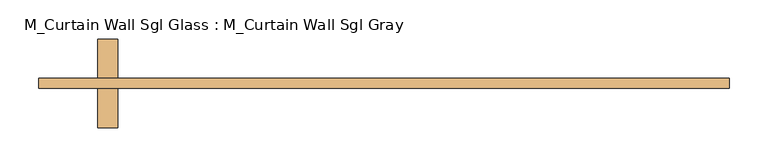
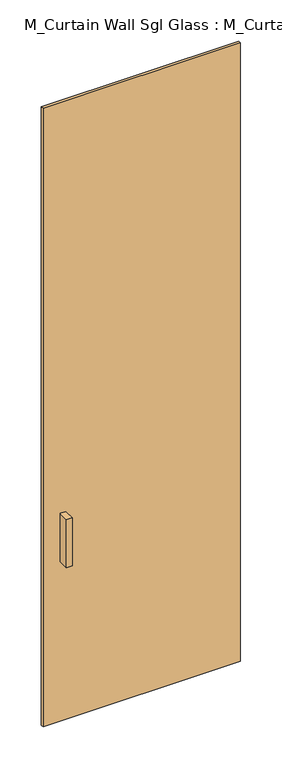
"""IFC4 building model written with IfcOpenShell, lengths in millimetres: door geometry, M_Curtain Wall Sgl Glass : M_Curtain Wall Sgl Gray."""

from ifc_helpers import new_model, si_unit, frame, origin, origin_with_axes, place, context, project, spatial, polyline, outline, extrude, source, transform, mapped, element, save


def m_curtain_wall_sgl_glass_m_curtain_wall_sgl_gray_2ca94d57(model_context):
    return source(origin(), model_context, "Body", "SweptSolid", [
        extrude(outline(polyline([(-343.4, -12.5), (-368.8, -12.5), (-368.8, 38.3), (-343.4, 38.3), (-343.4, -12.5)])), frame((0.0, 0.0, 762.0), z_axis=(0.0, 0.0, 1.0), x_axis=(1.0, 0.0, 0.0)), (0.0, 0.0, 1.0), 228.6),
        extrude(outline(polyline([(-368.8, 101.8), (-343.4, 101.8), (-343.4, 51.0), (-368.8, 51.0), (-368.8, 101.8)])), frame((0.0, 0.0, 762.0), z_axis=(0.0, 0.0, 1.0), x_axis=(1.0, 0.0, 0.0)), (0.0, 0.0, 1.0), 228.6),
        extrude(outline(polyline([(445.0, 51.0), (445.0, 38.3), (-445.0, 38.3), (-445.0, 51.0), (445.0, 51.0)])), origin_with_axes(), (0.0, 0.0, 1.0), 2950.0),
    ])


if __name__ == "__main__":
    model = new_model("IFC4")
    model_context = context("Model", 3, world=origin())
    ifc_project = project(units=[si_unit("LENGTHUNIT", "METRE", prefix="MILLI")], contexts=[model_context])
    site = spatial("IfcSite", under=ifc_project)
    building = spatial("IfcBuilding", under=site)
    placement = place(None, origin())
    m_curtain_wall_sgl_glass_m_curtain_wall_sgl_gray_shape = m_curtain_wall_sgl_glass_m_curtain_wall_sgl_gray_2ca94d57(model_context)
    element("IfcDoor", 1, ObjectType="M_Curtain Wall Sgl Glass : M_Curtain Wall Sgl Gray", at=placement, inside=building, context=model_context, shape_type="MappedRepresentation", body=[
        mapped(m_curtain_wall_sgl_glass_m_curtain_wall_sgl_gray_shape, transform((0.0, 0.0, 0.0), x_axis=(1.0, 0.0, 0.0), y_axis=(0.0, 1.0, 0.0), z_axis=(0.0, 0.0, 1.0))),
    ])
    save(model, "model.ifc")

# Revit data of these elements
# Type "M_Curtain Wall Sgl Glass : M_Curtain Wall Sgl Gray"
#   Model = "12345667"
#   Manufacturer = "Dublin Doors"
#   Description = "Single Flush door"
#   Type Mark = "48"
#   COBie.Type.CreatedBy = "design@eagle.com"
#   COBie.Type.CreatedOn = "2016-09-13T05:47:35"
#   COBie.Type.Name = "Doors_M_Curtain Wall Sgl Glass_M_Curtain Wall Sgl Gray"
#   COBie.Type.Category = "23-30 10 00 : Doors"
#   COBie.Type.Description = "Single Flush door"
#   COBie.Type.Manufacturer = "Dublin Doors"
#   COBie.Type.ModelNumber = "12345667"
#   Construction Type Id = "opn-d36"
#   Analytic Construction = "Wood panel"
#   COBie.Type.ReplacementCost = 0
#   Offset = 51 mm
#   Heat Transfer Coefficient (U) = 3.8042 W/(m²·K)
#   COBie.Type = yes
#   Function = 1
#   Glazing Material = Door - Frame(1)
#   Visual Light Transmittance = 0
#   Solar Heat Gain Coefficient = 0
# Element 1 (IfcDoor, "M_Curtain Wall Sgl Glass : M_Curtain Wall Sgl Gray")
#   Materials on its faces: "Aluminum", "Door - Frame(1)"
# Materials
#   "Door - Frame(1)": class "Miscellaneous", colour RGB 128 128 128, transparency 0, Cost = 0
#   "Aluminum": class "Metal", colour RGB 247 247 247, transparency 0, Description = "Aluminum 6061", Cost = 0
